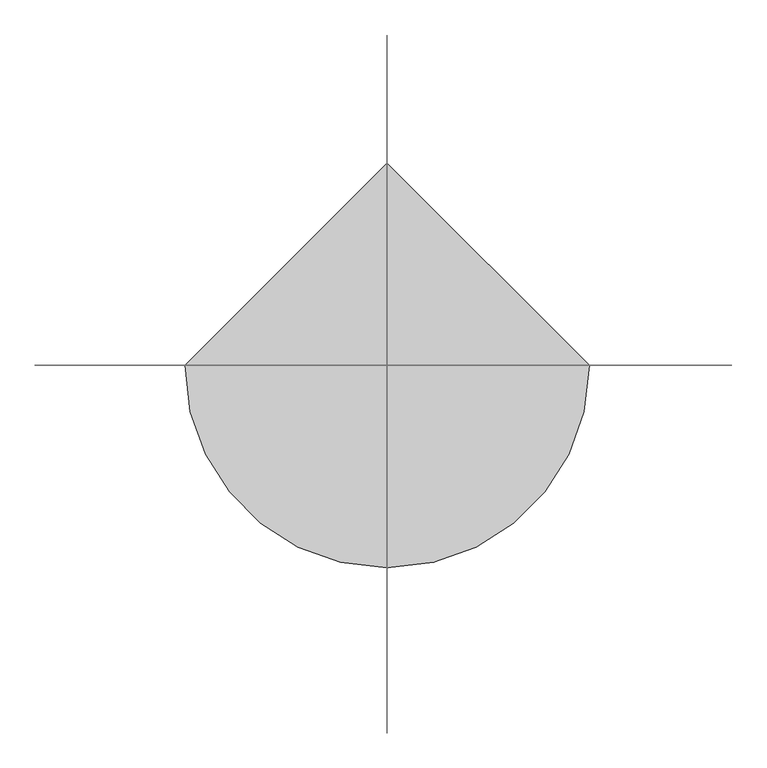
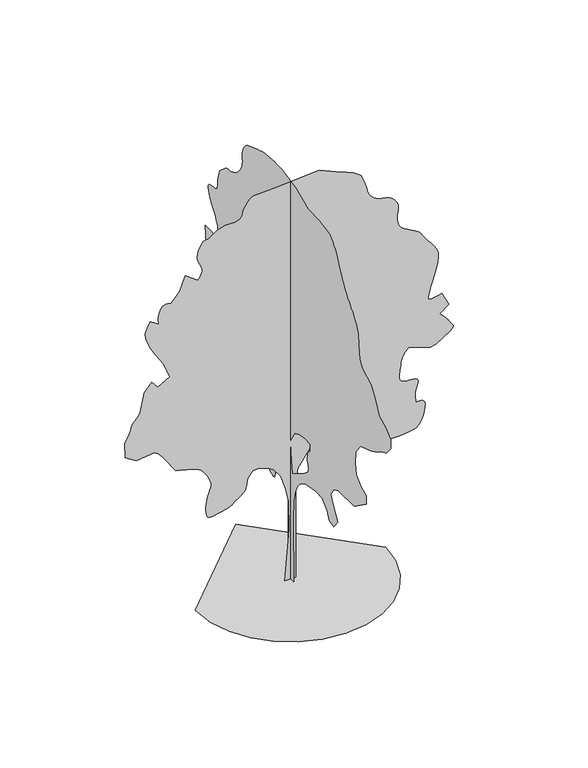
"""IFC4 building model written with IfcOpenShell, lengths in millimetres: geographic element geometry, RPC 木 - 落葉樹 : ポプラ - 7.6 メートル."""

from ifc_helpers import new_model, si_unit, origin, place, context, project, spatial, triangles, source, transform, mapped, element, save


def geographic_element_a2efc43f(model_context):
    return source(origin(), model_context, "Body", "Tessellation", [
        triangles([(92.8617737, 0.000406, 0.005513), (-103.915959, 0.000406, 0.005513), (-22.8901635, 0.0003494, 949.1680813), (-34.4652064, 0.0003176, 1481.626133), (-92.3406663, 0.0003011, 1759.4311237), (-173.3674883, 0.0002866, 2002.5093098), (-300.6936918, 0.0002762, 2176.1362118), (-404.8693279, 0.0002728, 2234.0127663), (-566.9214277, 0.0002694, 2291.8891754), (-682.6743914, 0.0002694, 2291.8891754), (-763.7004049, 0.0002762, 2176.1362118), (-798.427355, 0.0002852, 2025.6589142), (-801.2950579, 0.0002863, 2008.1460297), (-806.4934324, 0.0002874, 1989.7185207), (-816.3455927, 0.0002886, 1969.4722275), (-833.1871519, 0.0002899, 1946.489764), (-859.3387533, 0.0002915, 1919.8644997), (-897.1360102, 0.0002934, 1888.6816647), (-948.9046526, 0.0002956, 1852.0320122), (-998.3097038, 0.0002977, 1817.003627), (-1032.3247061, 0.0002993, 1790.0718407), (-1058.2431822, 0.0003005, 1769.4200489), (-1083.3510246, 0.0003015, 1753.2219097), (-1114.9365967, 0.0003023, 1739.6560226), (-1160.2933485, 0.000303, 1726.8980804), (-1226.7072453, 0.0003038, 1713.1294441), (-1299.8367931, 0.0003048, 1697.5064152), (-1361.0192505, 0.0003056, 1683.0943588), (-1411.0653236, 0.0003062, 1673.9514576), (-1450.7852829, 0.0003062, 1674.1187439), (-1480.9902706, 0.0003054, 1687.6517841), (-1502.4856155, 0.0003035, 1718.5964069), (-1516.0869656, 0.0003004, 1771.0059986), (-1522.0251205, 0.0002967, 1833.4043701), (-1521.0802654, 0.0002932, 1891.7521168), (-1514.8710514, 0.00029, 1946.2541679), (-1505.0164204, 0.0002869, 1997.1108021), (-1493.1376396, 0.0002841, 2044.5246231), (-1480.8535057, 0.0002815, 2088.6983803), (-1469.7852859, 0.000279, 2129.8370029), (-1458.1775642, 0.0002769, 2165.8103886), (-1444.9485752, 0.000275, 2196.5194153), (-1432.7328964, 0.0002733, 2225.2042923), (-1424.1600185, 0.0002715, 2255.1052288), (-1421.8648098, 0.0002695, 2289.4596725), (-1428.479377, 0.000267, 2331.5079781), (-1446.6356815, 0.0002638, 2384.4900639), (-1473.3978561, 0.0002604, 2441.7913628), (-1503.3976238, 0.0002573, 2494.2338013), (-1535.6266159, 0.0002545, 2541.2094223), (-1569.0690514, 0.0002521, 2582.1226227), (-1602.7142361, 0.00025, 2616.3228607), (-1635.5487144, 0.0002484, 2643.2520309), (-1666.5642632, 0.0002473, 2662.3026123), (-1701.7269424, 0.0002464, 2677.1732162), (-1746.6125748, 0.0002455, 2692.0694), (-1799.5946606, 0.0002446, 2706.940004), (-1859.0568741, 0.0002437, 2721.8358971), (-1923.3782387, 0.0002428, 2736.706501), (-1990.9396671, 0.000242, 2751.5771049), (-2060.1197468, 0.0002411, 2766.4732887), (-2256.8962532, 0.0002238, 3055.8556252), (-2301.7818855, 0.0002202, 3116.5289566), (-2338.160479, 0.0002175, 3161.4195305), (-2367.4508423, 0.0002156, 3193.1367805), (-2391.0741096, 0.0002144, 3214.3154297), (-2410.4440029, 0.0002136, 3227.61549), (-2426.9815109, 0.0002131, 3235.6461044), (-2442.1003555, 0.0002128, 3241.041996), (-2766.1945267, 0.0002148, 3206.3353935), (-2962.9836777, 0.0002073, 3333.6607613), (-2974.5611687, 0.0001914, 3599.8884064), (-2952.3436295, 0.000189, 3639.5351143), (-2930.8609291, 0.0001867, 3678.9789276), (-2910.7717484, 0.0001843, 3718.0428223), (-2892.8103447, 0.0001821, 3756.473616), (-2877.7118477, 0.0001798, 3794.0934128), (-2866.1343567, 0.0001776, 3830.70019), (-2858.8130013, 0.0001755, 3866.1160515), (-2847.3878265, 0.0001735, 3899.5814507), (-2825.6772331, 0.0001716, 3931.2481224), (-2797.4559906, 0.0001698, 3962.0787987), (-2766.6000252, 0.0001679, 3993.137368), (-2736.9852631, 0.000166, 4025.3865623), (-2712.4120537, 0.000164, 4059.8905609), (-2696.7560326, 0.0001617, 4097.611805), (-2627.2919586, 0.000141, 4444.881015), (-2488.4021805, 0.0001321, 4595.3354942), (-2384.2239464, 0.0001396, 4468.0101265), (-2164.2953648, 0.0001327, 4583.7832924), (-2280.0483284, 0.0001155, 4873.1403397), (-2465.2501053, 9.82e-05, 5162.5226761), (-2487.5231644, 9.58e-05, 5203.6643509), (-2513.036142, 9.27e-05, 5254.9385468), (-2539.3601166, 8.93e-05, 5312.268187), (-2564.0600624, 8.58e-05, 5371.6238663), (-2584.7067673, 8.24e-05, 5428.9535065), (-2598.8934013, 7.93e-05, 5480.2277023), (-2604.1628471, 7.69e-05, 5521.3693771), (-2601.4519661, 7.48e-05, 5555.7463486), (-2593.9027176, 7.28e-05, 5589.5407974), (-2582.2746483, 7.08e-05, 5622.8038834), (-2567.4293335, 6.89e-05, 5655.6611801), (-2550.1521904, 6.69e-05, 5688.2394241), (-2531.2585762, 6.5e-05, 5720.5903564), (-2511.5516396, 6.31e-05, 5752.8651306), (-2361.0744873, 6.93e-05, 5648.6941635), (-2365.8675087, 6.73e-05, 5681.019516), (-2369.6472198, 6.54e-05, 5713.8518143), (-2371.4003105, 6.34e-05, 5747.6968414), (-2370.118412, 6.13e-05, 5783.0621246), (-2364.7857433, 5.9e-05, 5820.4540283), (-2354.391465, 5.67e-05, 5860.3794983), (-2337.9248829, 5.41e-05, 5903.344899), (-2316.394075, 5.19e-05, 5940.9141174), (-2291.8258072, 5.04e-05, 5965.7155106), (-2264.7267345, 4.95e-05, 5979.8768555), (-2235.6036575, 4.92e-05, 5985.5515091), (-2204.9604698, 4.92e-05, 5984.8422501), (-2173.3064426, 4.95e-05, 5979.8768555), (-2141.1459057, 5e-05, 5972.7831024), (-1990.6686081, 3.96e-05, 6146.4178528), (-1886.4928448, 2.44e-05, 6401.0680069), (-1666.5642632, 3.41e-05, 6239.0110382), (-1644.4939533, 3.23e-05, 6268.8284042), (-1623.9409927, 3.05e-05, 6298.823085), (-1606.4256374, 2.87e-05, 6329.2229736), (-1593.4675621, 2.69e-05, 6360.2309647), (-1586.584552, 2.5e-05, 6392.0749512), (-1587.2913403, 2.3e-05, 6424.9066681), (-1597.1131245, 2.1e-05, 6458.9545898), (-1613.1085144, 1.89e-05, 6493.7879288), (-1630.1173599, 1.68e-05, 6529.2043716), (-1646.3153538, 1.46e-05, 6565.8614365), (-1659.8813862, 1.23e-05, 6604.3428085), (-1668.993766, 9.9e-06, 6645.2304291), (-1671.8286221, 7.3e-06, 6689.1585617), (-1666.5642632, 4.4e-06, 6736.759726), (-1653.9432312, 1.5e-06, 6785.3747818), (-1636.4607227, -1.2e-06, 6830.974324), (-1614.9299149, -3.6e-06, 6871.9131042), (-1590.1616592, -5.7e-06, 6906.5691284), (-1562.9612846, -7.3e-06, 6933.3209839), (-1534.1394974, -8.3e-06, 6950.5728378), (-1504.512236, -8.7e-06, 6956.6782791), (-1471.3382435, -9.2e-06, 6965.0132355), (-1431.8891979, -1.05e-05, 6986.521225), (-1386.9707188, -1.22e-05, 7015.9078033), (-1337.3959831, -1.41e-05, 7047.9291046), (-1283.9756973, -1.59e-05, 7077.315683), (-1227.5178062, -1.72e-05, 7098.8236725), (-1168.8306908, -1.77e-05, 7107.1580475), (-1109.0314339, -1.76e-05, 7106.8289978), (-1050.4481638, -1.77e-05, 7107.2847839), (-995.7104439, -1.79e-05, 7110.8060806), (-947.4530697, -1.84e-05, 7119.5718246), (-908.3054592, -1.94e-05, 7135.8353668), (-880.9024807, -2.09e-05, 7161.8273849), (-867.8760956, -2.32e-05, 7199.7512329), (-856.9422426, -2.61e-05, 7248.5941818), (-835.6824938, -2.93e-05, 7302.6804153), (-806.5264246, -3.26e-05, 7357.4009125), (-771.9008492, -3.56e-05, 7408.0420074), (-734.2403572, -3.81e-05, 7449.9940979), (-695.9718355, -3.98e-05, 7478.5696793), (-659.5247869, -4.04e-05, 7489.1335693), (-323.8458215, -4.18e-05, 7512.2885513), (509.5693688, -4.53e-05, 7570.1751343), (926.2744205, -3.42e-05, 7384.9631836), (995.3532709, -3.26e-05, 7357.5526474), (1062.2078384, -3.09e-05, 7329.4578506), (1124.6038118, -2.92e-05, 7299.9195374), (1180.3219225, -2.73e-05, 7268.2778641), (1227.1277138, -2.52e-05, 7233.7741562), (1262.7970482, -2.29e-05, 7195.7485703), (1285.1055702, -2.04e-05, 7153.4674301), (1299.9533558, -1.79e-05, 7111.9461273), (1314.5985374, -1.58e-05, 7075.1117477), (1328.8409821, -1.37e-05, 7040.480722), (1342.4753242, -1.16e-05, 7005.6473831), (1355.2991055, -9.4e-06, 6968.1799026), (1367.1094311, -6.8e-06, 6925.6702881), (1377.7063133, -3.9e-06, 6875.662294), (1393.5345623, -8e-07, 6823.9573105), (1419.2834267, 2e-06, 6778.1292938), (1452.117905, 4.3e-06, 6738.3811386), (1489.2059029, 6.3e-06, 6704.890741), (1527.709948, 7.9e-06, 6677.9104111), (1564.7979458, 9.1e-06, 6657.5936279), (1597.6348949, 9.9e-06, 6644.1415421), (1628.0070236, 1.04e-05, 6636.0856384), (1659.1872425, 1.07e-05, 6630.6638763), (1690.5726814, 1.1e-05, 6626.230426), (1721.5527672, 1.13e-05, 6621.2144531), (1751.5195427, 1.17e-05, 6613.9439667), (1779.8675217, 1.24e-05, 6602.8481323), (1805.9861309, 1.34e-05, 6586.2799576), (1831.2638031, 1.47e-05, 6563.7586578), (1856.5388592, 1.63e-05, 6536.6015945), (1880.3977226, 1.82e-05, 6505.7959167), (1901.4218754, 2.02e-05, 6472.3560974), (1918.1949795, 2.23e-05, 6437.2948654), (1929.2986622, 2.44e-05, 6401.625531), (1933.3139694, 2.65e-05, 6366.3364059), (1929.8053173, 2.9e-05, 6325.1191544), (1922.2457497, 3.2e-05, 6273.1351181), (1915.0916805, 3.56e-05, 6213.8805954), (1912.7964718, 3.93e-05, 6150.775145), (1919.8163921, 4.31e-05, 6087.2644867), (1940.6048035, 4.67e-05, 6026.7937592), (1979.615649, 5e-05, 5972.7831024), (2034.2165314, 5.26e-05, 5927.5631882), (2096.1082478, 5.5e-05, 5888.8289246), (2161.2401733, 5.71e-05, 5853.1340103), (2225.5615379, 5.92e-05, 5817.0088898), (2285.0238968, 6.16e-05, 5777.0584213), (2335.5764797, 6.44e-05, 5729.8118866), (2373.1711327, 6.79e-05, 5671.8491455), (2411.6421856, 7.17e-05, 5607.223439), (2462.6659607, 7.56e-05, 5541.7878983), (2518.9567108, 7.96e-05, 5474.7303635), (2573.2307236, 8.38e-05, 5405.2410004), (2618.1721664, 8.81e-05, 5332.5093933), (2646.5201454, 9.27e-05, 5255.7495438), (2650.9785942, 9.76e-05, 5174.0998764), (2634.6386032, 0.0001032, 5079.7841217), (2608.190799, 0.0001097, 4970.8762344), (2575.6628426, 0.0001165, 4855.508567), (2541.0826859, 0.0001233, 4741.7367325), (2508.5622871, 0.0001295, 4637.6927925), (2482.1043091, 0.0001347, 4551.4835197), (2465.7718758, 0.0001383, 4491.1648178), (2464.9611694, 0.0001404, 4454.9635391), (2480.5538223, 0.0001417, 4433.9369156), (2509.8113388, 0.0001422, 4425.5769608), (2550.0001648, 0.0001421, 4427.3248192), (2598.3867462, 0.0001415, 4436.6727951), (2652.2453773, 0.0001407, 4451.0876129), (2708.839888, 0.0001396, 4468.0101265), (2836.1652557, 0.0001548, 4213.3596817), (2674.1332855, 0.0001624, 4086.0346046), (2698.8841003, 0.0001637, 4063.6400414), (2723.4573097, 0.0001651, 4040.7132431), (2747.6253113, 0.0001665, 4016.7987144), (2771.1852104, 0.0001681, 3991.3386406), (2793.9344032, 0.0001697, 3963.8772354), (2815.6705765, 0.0001715, 3933.8828453), (2836.1652557, 0.0001735, 3900.8482338), (2858.1037422, 0.0001754, 3868.6749069), (2881.2584335, 0.000177, 3840.554821), (2901.1702995, 0.0001786, 3814.8921432), (2913.3811821, 0.0001801, 3790.0148827), (2913.4570496, 0.0001816, 3764.3269157), (2896.9144547, 0.0001833, 3736.232119), (2859.3199471, 0.0001852, 3704.0590828), (2604.6695023, 0.0001955, 3530.4243324), (2500.4962097, 0.0001962, 3518.8471321), (2118.5182171, 0.0001886, 3646.1722092), (2091.3836815, 0.0001903, 3618.7110947), (2065.163625, 0.000192, 3590.1349319), (2040.7651142, 0.0001938, 3559.3298355), (2019.0975414, 0.0001958, 3525.1551773), (2001.0780018, 0.0001981, 3486.5726486), (1987.6134167, 0.0002008, 3442.3913338), (1979.615649, 0.0002038, 3391.5220551), (1974.0473843, 0.0002068, 3342.1474525), (1967.6684132, 0.0002092, 3301.2848305), (1961.0868382, 0.0002113, 3266.096862), (1954.9106163, 0.0002132, 3233.7206406), (1949.7477047, 0.0002151, 3201.3699989), (1946.2035896, 0.0002172, 3166.1567413), (1944.888699, 0.0002197, 3125.2941193), (1953.8643139, 0.000222, 3086.7368797), (1977.0163891, 0.0002236, 3059.0981598), (2008.6704163, 0.0002247, 3040.5542336), (2043.1591541, 0.0002254, 3029.3316628), (2074.8131813, 0.0002257, 3023.5555618), (2097.9652565, 0.0002259, 3021.4277847), (2106.9408714, 0.0002259, 3021.1237335), (2119.5973663, 0.0002258, 3022.0103073), (2151.4868443, 0.0002258, 3022.4663841), (2193.5021576, 0.000226, 3019.2997169), (2236.5307812, 0.0002266, 3009.2421913), (2271.4578644, 0.0002278, 2989.0771431), (2289.1759689, 0.0002298, 2955.5102966), (2280.5702442, 0.0002328, 2905.3758568), (2259.8146797, 0.0002362, 2847.8691925), (2246.3499493, 0.0002394, 2794.0105614), (2238.9578133, 0.0002425, 2743.191861), (2236.4270084, 0.0002453, 2694.7799904), (2237.5416206, 0.0002481, 2648.2174255), (2241.0857357, 0.0002508, 2602.8707748), (2245.8432941, 0.0002535, 2558.1066467), (2285.1910378, 0.0002532, 2562.540097), (2322.5171024, 0.0002531, 2563.730722), (2355.7899261, 0.0002535, 2558.4106979), (2382.9903008, 0.0002544, 2543.4133575), (2402.0916058, 0.000256, 2515.4278564), (2411.0672207, 0.0002587, 2471.2540993), (2407.8954666, 0.0002625, 2407.6395229), (2395.1731327, 0.0002668, 2334.9507912), (2376.9836906, 0.0002708, 2266.9155544), (2353.5301804, 0.0002745, 2205.3632069), (2325.0124443, 0.0002777, 2152.110062), (2291.6383186, 0.0002803, 2108.9801365), (2253.6054657, 0.0002821, 2077.7999176), (2211.1189602, 0.0002832, 2060.3858643), (2171.2620907, 0.0002837, 2051.7801395), (2137.4826118, 0.000284, 2045.4011684), (2104.5113686, 0.0002843, 2040.64361), (2067.0864727, 0.0002845, 2036.8967457), (2019.9412399, 0.0002847, 2033.5578506), (1957.8137821, 0.000285, 2030.0137356), (1875.4374149, 0.0002852, 2025.6589142), (1785.9069786, 0.0002851, 2027.1105698), (1704.880965, 0.0002844, 2040.1039627), (1630.9405655, 0.000283, 2062.7139198), (1562.6724941, 0.0002812, 2093.0175934), (1498.6551807, 0.0002791, 2129.0947517), (1437.4727234, 0.0002767, 2169.0176056), (1377.7063133, 0.0002742, 2210.8631618), (1123.0508543, 0.0002597, 2453.9412025), (856.8231365, 0.0002528, 2569.6841377), (544.2937391, 0.0002542, 2546.5547356), (393.8164052, 0.0002611, 2430.7917435), (289.6407691, 0.00027, 2280.3144459), (127.5871523, 0.0002838, 2048.8109894), (92.8617737, 0.0003011, 1759.4311237), (92.8617737, 0.0003383, 1134.3723289), (-0.0023646, 90.6053344, 1.1e-05), (-0.0023646, -94.5971056, 0.0), (-0.0023646, -83.0220672, 1157.5168465), (-0.0023646, -94.5971056, 1527.9227257), (-0.0023646, -140.8980313, 1724.6992321), (-0.0023646, -210.3490428, 1875.1765297), (-0.0023646, -302.9508941, 1990.9294933), (-0.0023646, -441.8534077, 2071.9555069), (-0.0023646, -557.6038279, 2095.1051113), (-0.0023646, -789.1072117, 2141.4067909), (-0.0023646, -985.8861889, 2129.8320614), (-0.0023646, -1136.3635592, 1979.3546185), (-0.0023646, -1205.8147705, 1840.4521957), (-0.0023646, -1333.1399929, 1794.1505161), (-0.0023646, -1472.042561, 1967.7774181), (-0.0023646, -1321.5652634, 2199.2832001), (-0.0023646, -1252.1139793, 2361.3353725), (-0.0023646, -1333.1399929, 2500.2354698), (-0.0023646, -1483.6172905, 2569.6841377), (-0.0023646, -1969.7736626, 2569.6841377), (-0.0023646, -2351.7542713, 2835.9117828), (-0.0023646, -2351.7542713, 2997.9690422), (-0.0023646, -2189.7022442, 3067.4075363), (-0.0023646, -2039.2249466, 3206.3101044), (-0.0023646, -2004.5004673, 3403.0992554), (-0.0023646, -2027.6500717, 3634.5950089), (-0.0023646, -2178.1273693, 3831.3841599), (-0.0023646, -2444.3551598, 3923.9773453), (-0.0023646, -2488.9367409, 3941.4068047), (-0.0023646, -2533.110498, 3959.1147354), (-0.0023646, -2576.4735489, 3977.4307686), (-0.0023646, -2618.6279526, 3996.6839539), (-0.0023646, -2659.1612343, 4017.1280548), (-0.0023646, -2697.6678955, 4039.0918304), (-0.0023646, -2733.7427284, 4062.8799133), (-0.0023646, -2768.4493309, 4086.3386559), (-0.0023646, -2803.1812225, 4107.3652794), (-0.0023646, -2837.9131142, 4126.3652824), (-0.0023646, -2872.6450058, 4143.7438728), (-0.0023646, -2907.351899, 4159.9065491), (-0.0023646, -2942.0837906, 4175.258519), (-0.0023646, -2976.8156822, 4190.2052811), (-0.0023646, -3104.1407593, 4352.2622498), (-0.0023646, -3104.1407593, 4514.3195091), (-0.0023646, -2953.6609909, 4653.2220772), (-0.0023646, -2756.8971291, 4757.3924629), (-0.0023646, -2629.5467628, 5000.4657074), (-0.0023646, -2502.234185, 5185.6776581), (-0.0023646, -2224.4290489, 5336.1574265), (-0.0023646, -2143.4030354, 5463.4827942), (-0.0023646, -2120.2509602, 5718.1329483), (-0.0023646, -2097.1013557, 5926.4743011), (-0.0023646, -2072.264645, 5978.4327576), (-0.0023646, -2047.225185, 6029.4540619), (-0.0023646, -2021.7779011, 6078.651059), (-0.0023646, -1995.7251308, 6125.1127579), (-0.0023646, -1968.8641251, 6167.9514221), (-0.0023646, -1940.9873383, 6206.2043198), (-0.0023646, -1911.8997242, 6239.0110382), (-0.0023646, -1875.8225658, 6277.7964615), (-0.0023646, -1830.2327614, 6330.9455429), (-0.0023646, -1779.7788643, 6393.0121033), (-0.0023646, -1729.1274502, 6458.4988037), (-0.0023646, -1682.9270725, 6521.9838821), (-0.0023646, -1645.83922, 6577.9705811), (-0.0023646, -1622.5198586, 6620.9865601), (-0.0023646, -1605.6807701, 6657.1372604), (-0.0023646, -1585.6016178, 6696.1255783), (-0.0023646, -1563.2930958, 6737.9253525), (-0.0023646, -1539.7736012, 6782.5877426), (-0.0023646, -1516.0490318, 6830.0627518), (-0.0023646, -1493.1350235, 6880.3742157), (-0.0023646, -1472.042561, 6933.5238785), (-0.0023646, -1448.8245014, 6986.749118), (-0.0023646, -1419.5316673, 7037.5425293), (-0.0023646, -1385.1770782, 7086.3087387), (-0.0023646, -1346.7743351, 7133.4541168), (-0.0023646, -1305.3316612, 7179.3832901), (-0.0023646, -1261.8673084, 7224.5020477), (-0.0023646, -1217.3895727, 7269.2155975), (-0.0023646, -893.2828297, 7327.0766006), (-0.0023646, -546.029062, 7338.653801), (-0.0023646, -175.623419, 7500.711351), (-0.0023646, 264.2314734, 7593.3045364), (-0.0023646, 323.6937959, 7595.7363647), (-0.0023646, 382.7508016, 7597.8641418), (-0.0023646, 440.9996807, 7599.3843979), (-0.0023646, 498.0300296, 7599.9925003), (-0.0023646, 553.4441254, 7599.3843979), (-0.0023646, 606.831528, 7597.2566208), (-0.0023646, 657.7895004, 7593.3045364), (-0.0023646, 706.7891258, 7588.2379852), (-0.0023646, 754.9781902, 7582.5883301), (-0.0023646, 802.9670488, 7575.6974716), (-0.0023646, 851.3612606, 7566.9828873), (-0.0023646, 900.7663118, 7555.8620544), (-0.0023646, 951.7900869, 7541.6751297), (-0.0023646, 1005.0432318, 7523.8657516), (-0.0023646, 1340.7248497, 7408.1181656), (-0.0023646, 1370.3545818, 7383.1138779), (-0.0023646, 1399.173753, 7356.8683868), (-0.0023646, 1426.3741276, 7328.2166473), (-0.0023646, 1451.1425285, 7295.9418732), (-0.0023646, 1472.6733364, 7258.7778625), (-0.0023646, 1490.1558449, 7215.5595703), (-0.0023646, 1502.7768768, 7165.019632), (-0.0023646, 1507.1292274, 7116.7342072), (-0.0023646, 1503.584967, 7077.7714691), (-0.0023646, 1497.0060081, 7043.2421814), (-0.0023646, 1492.2458336, 7008.3076859), (-0.0023646, 1494.1711521, 6968.128743), (-0.0023646, 1507.6358826, 6917.7916992), (-0.0023646, 1537.5012108, 6852.5078934), (-0.0023646, 1578.4019119, 6786.1851974), (-0.0023646, 1620.9238804, 6734.4546341), (-0.0023646, 1663.8485859, 6694.8587952), (-0.0023646, 1705.9652012, 6664.9908508), (-0.0023646, 1746.0576668, 6642.4189728), (-0.0023646, 1782.9075977, 6624.7107513), (-0.0023646, 1815.3063469, 6609.4093597), (-0.0023646, 1845.0703732, 6598.3135254), (-0.0023646, 1874.8345448, 6592.8923447), (-0.0023646, 1904.598571, 6590.2826202), (-0.0023646, 1934.3652134, 6587.6984756), (-0.0023646, 1964.129385, 6582.2522964), (-0.0023646, 1993.8934113, 6571.1558807), (-0.0023646, 2023.6575829, 6551.5483566), (-0.0023646, 2197.2869556, 6401.0680069), (-0.0023646, 2266.7357689, 6181.1500351), (-0.0023646, 2264.4760231, 6146.5445892), (-0.0023646, 2263.5310226, 6112.7751389), (-0.0023646, 2265.2182743, 6080.6021027), (-0.0023646, 2270.8549942, 6050.8858932), (-0.0023646, 2281.7533115, 6024.3875107), (-0.0023646, 2299.23582, 6001.9417877), (-0.0023646, 2324.612178, 5984.3608841), (-0.0023646, 2359.9116222, 5974.3033585), (-0.0023646, 2402.9047829, 5970.5285889), (-0.0023646, 2448.5301956, 5967.9700241), (-0.0023646, 2491.7284309, 5961.5605316), (-0.0023646, 2527.4306122, 5946.2341415), (-0.0023646, 2550.5826874, 5916.92314), (-0.0023646, 2556.1053154, 5868.6127167), (-0.0023646, 2547.4413094, 5812.448703), (-0.0023646, 2532.0893394, 5762.3651321), (-0.0023646, 2511.1641632, 5717.3475311), (-0.0023646, 2485.7878052, 5676.3837524), (-0.0023646, 2457.0700813, 5638.4599045), (-0.0023646, 2426.1228424, 5602.562677), (-0.0023646, 2394.0634621, 5567.6531799), (-0.0023646, 2369.3609001, 5525.4981949), (-0.0023646, 2345.2664406, 5483.4705276), (-0.0023646, 2322.3854244, 5441.6201752), (-0.0023646, 2301.3284248, 5400.0732925), (-0.0023646, 2282.698312, 5358.9321991), (-0.0023646, 2267.1081299, 5318.2974701), (-0.0023646, 2255.160894, 5278.2708435), (-0.0023646, 2248.95168, 5240.6254669), (-0.0023646, 2249.4254883, 5206.6025436), (-0.0023646, 2255.4649452, 5175.6201324), (-0.0023646, 2265.9605255, 5147.0695496), (-0.0023646, 2279.797617, 5120.3426926), (-0.0023646, 2295.861462, 5094.8320404), (-0.0023646, 2313.0374485, 5069.9294907), (-0.0023646, 2463.5147461, 5093.0844727), (-0.0023646, 2648.7240807, 5093.0844727), (-0.0023646, 2625.5693893, 4757.3924629), (-0.0023646, 2417.2130665, 4398.5716324), (-0.0023646, 2409.7574169, 4356.4422272), (-0.0023646, 2402.1979946, 4314.642453), (-0.0023646, 2394.4358231, 4273.4252014), (-0.0023646, 2386.3697456, 4233.1451019), (-0.0023646, 2377.898315, 4194.0559181), (-0.0023646, 2368.9227001, 4156.486409), (-0.0023646, 2359.3391281, 4120.7664963), (-0.0023646, 2344.9953815, 4082.1586784), (-0.0023646, 2323.9712288, 4037.2681046), (-0.0023646, 2299.5044083, 3988.3492882), (-0.0023646, 2274.8373093, 3937.5814568), (-0.0023646, 2253.2051994, 3887.2441223), (-0.0023646, 2237.8507587, 3839.5162216), (-0.0023646, 2232.0114349, 3796.6522682), (-0.0023646, 2236.7360012, 3758.6522621), (-0.0023646, 2249.9651356, 3723.6921867), (-0.0023646, 2270.279884, 3691.2656776), (-0.0023646, 2296.2641991, 3660.865789), (-0.0023646, 2326.5020336, 3631.9602859), (-0.0023646, 2359.5747242, 3604.0936729), (-0.0023646, 2394.0634621, 3576.7337151), (-0.0023646, 2706.5853745, 3646.1722092), (-0.0023646, 2723.8372284, 3596.6458717), (-0.0023646, 2740.3798233, 3547.4991623), (-0.0023646, 2755.5039001, 3499.1884483), (-0.0023646, 2768.4746201, 3452.0686501), (-0.0023646, 2778.6333023, 3406.5699738), (-0.0023646, 2785.245108, 3363.0979179), (-0.0023646, 2787.6266487, 3322.0832703), (-0.0023646, 2774.199852, 3282.9940865), (-0.0023646, 2739.6958534, 3244.7153183), (-0.0023646, 2692.8545265, 3206.6647339), (-0.0023646, 2642.3654572, 3168.1833618), (-0.0023646, 2596.9426483, 3128.7142593), (-0.0023646, 2565.3015564, 3087.5981644), (-0.0023646, 2556.1053154, 3044.2784248), (-0.0023646, 2564.4399811, 3002.6556747), (-0.0023646, 2578.8547989, 2966.5049744), (-0.0023646, 2598.3361679, 2934.9397499), (-0.0023646, 2621.8454887, 2906.9969788), (-0.0023646, 2648.4200294, 2881.7903778), (-0.0023646, 2676.9959015, 2858.3825043), (-0.0023646, 2706.5853745, 2835.9117828), (-0.0023646, 2776.0491577, 2604.4160294), (-0.0023646, 2709.3974121, 2602.1106468), (-0.0023646, 2644.670549, 2600.945311), (-0.0023646, 2583.7946136, 2601.984201), (-0.0023646, 2528.6796638, 2606.3667824), (-0.0023646, 2481.2656975, 2615.2081032), (-0.0023646, 2443.468586, 2629.6226303), (-0.0023646, 2417.2130665, 2650.725412), (-0.0023646, 2391.9710026, 2676.8694557), (-0.0023646, 2357.0109272, 2705.4453278), (-0.0023646, 2313.9494568, 2736.0478203), (-0.0023646, 2264.407568, 2768.2973053), (-0.0023646, 2210.0068188, 2801.7371246), (-0.0023646, 2152.3684765, 2835.987941), (-0.0023646, 2093.1088669, 2870.6436745), (-0.0023646, 2090.6463718, 2833.3785072), (-0.0023646, 2088.2828533, 2795.8345779), (-0.0023646, 2086.1244095, 2757.6572571), (-0.0023646, 2084.2675461, 2718.5680733), (-0.0023646, 2082.8158905, 2678.2879738), (-0.0023646, 2081.8710354, 2636.4626198), (-0.0023646, 2081.533992, 2592.838829), (-0.0023646, 2079.9481876, 2547.390731), (-0.0023646, 2074.514217, 2502.7332825), (-0.0023646, 2064.2212406, 2462.5418404), (-0.0023646, 2048.0560936, 2430.4471424), (-0.0023646, 2025.0077911, 2410.0994019), (-0.0023646, 1994.0631683, 2405.1366234), (-0.0023646, 1954.2062988, 2419.2093109), (-0.0023646, 1909.2219807, 2445.3635284), (-0.0023646, 1863.6321762, 2473.9469582), (-0.0023646, 1817.5331005, 2504.5546829), (-0.0023646, 1771.028817, 2536.7762627), (-0.0023646, 1724.222953, 2570.216082), (-0.0023646, 1677.2144852, 2604.4921875), (-0.0023646, 1630.1020992, 2639.147921), (-0.0023646, 1352.2995792, 2720.1639061), (-0.0023646, 1074.4945158, 2627.5707207), (-0.0023646, 900.8676138, 2419.2093109), (-0.0023646, 923.2419748, 2389.5794334), (-0.0023646, 945.9203871, 2360.7602623), (-0.0023646, 969.204213, 2333.5598877), (-0.0023646, 993.4000471, 2308.7914867), (-0.0023646, 1018.8119408, 2287.2608242), (-0.0023646, 1045.7412563, 2269.7783157), (-0.0023646, 1074.4945158, 2257.1571384), (-0.0023646, 1101.897567, 2244.8731499), (-0.0023646, 1125.0471714, 2228.3379673), (-0.0023646, 1144.6551315, 2208.258815), (-0.0023646, 1161.4257648, 2185.344952), (-0.0023646, 1176.07349, 2160.305492), (-0.0023646, 1189.3025517, 2133.8473686), (-0.0023646, 1201.8222816, 2106.6798409), (-0.0023646, 1169.4919149, 2099.1888737), (-0.0023646, 1136.6573639, 2091.3937099), (-0.0023646, 1102.8070318, 2082.9907345), (-0.0023646, 1067.4417486, 2073.6756054), (-0.0023646, 1030.0497723, 2063.1471783), (-0.0023646, 990.1269911, 2051.0986404), (-0.0023646, 947.16675, 2037.2285568), (-0.0023646, 904.2091249, 2020.3237747), (-0.0023646, 864.2863438, 1999.7708141), (-0.0023646, 826.8943674, 1976.1830097), (-0.0023646, 791.5265408, 1950.1630863), (-0.0023646, 757.6786795, 1922.3217625), (-0.0023646, 724.8442011, 1893.2645245), (-0.0023646, 692.5138344, 1863.6018002), (-0.0023646, 692.5138344, 1701.5496277), (-0.0023646, 650.5998957, 1674.7216141), (-0.0023646, 610.2059223, 1650.6246838), (-0.0023646, 572.8469018, 1631.9970417), (-0.0023646, 540.0453429, 1621.5699165), (-0.0023646, 513.3187039, 1622.0765717), (-0.0023646, 494.1844431, 1636.2505611), (-0.0023646, 484.160055, 1666.8252937), (-0.0023646, 479.2682024, 1701.4811726), (-0.0023646, 474.7791232, 1728.6487003), (-0.0023646, 471.100714, 1752.1706657), (-0.0023646, 468.638328, 1775.8927643), (-0.0023646, 467.7947385, 1803.6682491), (-0.0023646, 468.9752624, 1839.3374382), (-0.0023646, 472.5852528, 1886.7512592), (-0.0023646, 475.5213744, 1938.6212036), (-0.0023646, 474.8120427, 1985.6298168), (-0.0023646, 471.0677945, 2028.5899853), (-0.0023646, 464.8915363, 2068.3100899), (-0.0023646, 456.893805, 2105.6006916), (-0.0023646, 447.6800869, 2141.2724968), (-0.0023646, 437.8608825, 2176.1311249), (-0.0023646, 241.0823958, 2187.7059998), (-0.0023646, 136.90626, 1990.9294933), (-0.0023646, 79.030296, 1655.2479481), (-0.0023646, 79.030296, 1226.9681305), (-0.0023646, 79.030296, 590.3344608), (-0.0022449, -48.2969385, 2025.6538273), (-0.0022449, -1.9959556, 2396.0597065), (-0.0022449, 9.5791312, 2615.9935204), (-0.0022449, -129.3229929, 2835.9117828), (-0.0022449, -279.801326, 2905.3758568), (-0.0022449, -453.4282099, 2928.5049683), (-0.0022449, -615.4803097, 2928.5049683), (-0.0022449, -615.4803097, 2789.62798), (-0.0022449, -534.4542598, 2720.1639061), (-0.0022449, -511.3046917, 2558.1066467), (-0.0022449, -521.1568156, 2548.0241226), (-0.0022449, -530.6061298, 2536.9279976), (-0.0022449, -539.2448104, 2523.7927528), (-0.0022449, -546.6699749, 2507.6277512), (-0.0022449, -552.4738358, 2487.4115433), (-0.0022449, -556.2535832, 2462.1366325), (-0.0022449, -557.6038279, 2430.7840405), (-0.0022449, -554.2294335, 2398.4207542), (-0.0022449, -544.7801193, 2370.3109875), (-0.0022449, -530.2691955, 2345.7427197), (-0.0022449, -511.7075014, 2324.0093079), (-0.0022449, -490.1108545, 2304.4038185), (-0.0022449, -466.4875508, 2286.2145218), (-0.0022449, -441.8534077, 2268.7320133), (-1707.3661331, 0.0, 0.0031185), (-1662.2297894, -391.2146745, 0.0030952), (-1533.678479, -750.4840605, 0.0030738), (-1332.01012, -1067.5126745, 0.0030549), (-1067.5126745, -1332.01012, 0.0030391), (-750.4840605, -1533.678479, 0.0030271), (-391.2146745, -1662.2297894, 0.0030194), (7.48e-05, -1707.3661331, 0.0030167), (391.2146745, -1662.2297894, 0.0030194), (750.4840605, -1533.678479, 0.0030271), (1067.5126745, -1332.01012, 0.0030391), (1332.01012, -1067.5126745, 0.0030549), (1533.678479, -750.4840605, 0.0030738), (1662.2297894, -391.2146745, 0.0030952), (1707.3661331, 0.0001493, 0.0031185), (-0.0002245, 1707.3661331, 0.0032203)], [[122, 123, 124], [87, 88, 89], [1, 2, 3], [329, 1, 3], [329, 3, 4], [328, 329, 4], [328, 4, 5], [105, 106, 107], [327, 328, 5], [327, 5, 6], [104, 105, 107], [238, 239, 240], [238, 240, 241], [237, 238, 241], [236, 237, 241], [103, 104, 107], [86, 87, 89], [235, 236, 241], [102, 103, 107], [101, 102, 107], [100, 101, 107], [99, 100, 107], [98, 99, 107], [97, 98, 107], [96, 97, 107], [327, 6, 7], [326, 327, 7], [95, 96, 107], [70, 71, 72], [69, 70, 72], [69, 72, 73], [69, 73, 74], [69, 74, 75], [69, 75, 76], [69, 76, 77], [69, 77, 78], [94, 95, 107], [234, 235, 241], [93, 94, 107], [69, 78, 79], [69, 79, 80], [69, 80, 81], [69, 81, 82], [69, 82, 83], [69, 83, 84], [69, 84, 85], [68, 69, 85], [325, 326, 7], [325, 7, 8], [67, 68, 85], [92, 93, 107], [91, 92, 107], [60, 61, 62], [67, 85, 86], [67, 86, 89], [67, 89, 90], [66, 67, 90], [65, 66, 90], [64, 65, 90], [63, 64, 90], [62, 63, 90], [60, 62, 90], [59, 60, 90], [58, 59, 90], [57, 58, 90], [56, 57, 90], [55, 56, 90], [54, 55, 90], [53, 54, 90], [284, 285, 286], [283, 284, 286], [282, 283, 286], [282, 286, 287], [281, 282, 287], [280, 281, 287], [279, 280, 287], [279, 287, 288], [278, 279, 288], [277, 278, 288], [277, 288, 289], [276, 277, 289], [275, 276, 289], [275, 289, 290], [52, 53, 90], [325, 8, 9], [121, 122, 124], [275, 290, 291], [30, 31, 32], [29, 30, 32], [29, 32, 33], [28, 29, 33], [28, 33, 34], [27, 28, 34], [27, 34, 35], [27, 35, 36], [26, 27, 36], [26, 36, 37], [26, 37, 38], [25, 26, 38], [25, 38, 39], [24, 25, 39], [23, 24, 39], [22, 23, 39], [21, 22, 39], [20, 21, 39], [20, 39, 40], [20, 40, 41], [20, 41, 42], [19, 20, 42], [19, 42, 43], [18, 19, 43], [18, 43, 44], [17, 18, 44], [16, 17, 44], [15, 16, 44], [14, 15, 44], [13, 14, 44], [12, 13, 44], [11, 12, 44], [11, 44, 45], [11, 45, 46], [10, 11, 46], [10, 46, 47], [10, 47, 48], [10, 48, 49], [10, 49, 50], [10, 50, 51], [252, 253, 254], [251, 252, 254], [251, 254, 255], [250, 251, 255], [249, 250, 255], [249, 255, 256], [248, 249, 256], [247, 248, 256], [246, 247, 256], [245, 246, 256], [245, 256, 257], [245, 257, 258], [244, 245, 258], [243, 244, 258], [242, 243, 258], [241, 242, 258], [234, 241, 258], [233, 234, 258], [274, 275, 291], [324, 325, 9], [51, 52, 90], [10, 51, 90], [9, 10, 90], [324, 9, 90], [323, 324, 90], [323, 90, 91], [323, 91, 107], [323, 107, 108], [323, 108, 109], [323, 109, 110], [323, 110, 111], [323, 111, 112], [323, 112, 113], [323, 113, 114], [323, 114, 115], [323, 115, 116], [323, 116, 117], [323, 117, 118], [323, 118, 119], [323, 119, 120], [323, 120, 121], [323, 121, 124], [323, 124, 125], [323, 125, 126], [323, 126, 127], [323, 127, 128], [323, 128, 129], [322, 323, 129], [322, 129, 130], [167, 168, 169], [274, 291, 292], [296, 297, 298], [296, 298, 299], [295, 296, 299], [294, 295, 299], [294, 299, 300], [293, 294, 300], [293, 300, 301], [293, 301, 302], [293, 302, 303], [293, 303, 304], [293, 304, 305], [293, 305, 306], [293, 306, 307], [293, 307, 308], [293, 308, 309], [293, 309, 310], [293, 310, 311], [293, 311, 312], [293, 312, 313], [293, 313, 314], [293, 314, 315], [293, 315, 316], [293, 316, 317], [293, 317, 318], [293, 318, 319], [292, 293, 319], [274, 292, 319], [274, 319, 320], [274, 320, 321], [274, 321, 322], [273, 274, 322], [273, 322, 130], [272, 273, 130], [271, 272, 130], [270, 271, 130], [269, 270, 130], [268, 269, 130], [267, 268, 130], [266, 267, 130], [265, 266, 130], [264, 265, 130], [263, 264, 130], [262, 263, 130], [261, 262, 130], [260, 261, 130], [259, 260, 130], [258, 259, 130], [233, 258, 130], [232, 233, 130], [231, 232, 130], [230, 231, 130], [229, 230, 130], [228, 229, 130], [227, 228, 130], [226, 227, 130], [225, 226, 130], [224, 225, 130], [223, 224, 130], [222, 223, 130], [221, 222, 130], [220, 221, 130], [219, 220, 130], [218, 219, 130], [217, 218, 130], [216, 217, 130], [215, 216, 130], [214, 215, 130], [213, 214, 130], [212, 213, 130], [211, 212, 130], [210, 211, 130], [209, 210, 130], [208, 209, 130], [207, 208, 130], [206, 207, 130], [205, 206, 130], [204, 205, 130], [203, 204, 130], [202, 203, 130], [201, 202, 130], [200, 201, 130], [199, 200, 130], [198, 199, 130], [197, 198, 130], [196, 197, 130], [195, 196, 130], [194, 195, 130], [193, 194, 130], [192, 193, 130], [191, 192, 130], [190, 191, 130], [189, 190, 130], [188, 189, 130], [187, 188, 130], [186, 187, 130], [185, 186, 130], [184, 185, 130], [183, 184, 130], [182, 183, 130], [181, 182, 130], [180, 181, 130], [179, 180, 130], [178, 179, 130], [177, 178, 130], [176, 177, 130], [175, 176, 130], [174, 175, 130], [173, 174, 130], [172, 173, 130], [171, 172, 130], [170, 171, 130], [169, 170, 130], [167, 169, 130], [167, 130, 131], [167, 131, 132], [167, 132, 133], [167, 133, 134], [167, 134, 135], [167, 135, 136], [164, 165, 166], [164, 166, 167], [163, 164, 167], [162, 163, 167], [161, 162, 167], [160, 161, 167], [159, 160, 167], [158, 159, 167], [143, 144, 145], [142, 143, 145], [141, 142, 145], [140, 141, 145], [140, 145, 146], [139, 140, 146], [138, 139, 146], [137, 138, 146], [136, 137, 146], [136, 146, 147], [136, 147, 148], [136, 148, 149], [136, 149, 150], [136, 150, 151], [136, 151, 152], [136, 152, 153], [136, 153, 154], [136, 154, 155], [136, 155, 156], [157, 158, 167], [157, 167, 136], [157, 136, 156], [634, 330, 635], [633, 634, 635], [632, 633, 635], [631, 632, 635], [540, 541, 542], [592, 593, 594], [494, 495, 496], [635, 330, 331], [635, 331, 332], [635, 332, 333], [635, 333, 334], [635, 334, 335], [658, 635, 335], [658, 335, 336], [658, 336, 337], [658, 337, 338], [540, 542, 543], [657, 658, 338], [631, 635, 636], [630, 631, 636], [518, 519, 520], [656, 657, 338], [656, 338, 339], [655, 656, 339], [654, 655, 339], [653, 654, 339], [540, 543, 544], [539, 540, 544], [518, 520, 521], [539, 544, 545], [538, 539, 545], [538, 545, 546], [538, 546, 547], [538, 547, 548], [537, 538, 548], [537, 548, 549], [536, 537, 549], [536, 549, 550], [536, 550, 551], [535, 536, 551], [535, 551, 552], [534, 535, 552], [493, 494, 496], [493, 496, 497], [343, 344, 345], [342, 343, 345], [341, 342, 345], [340, 341, 345], [340, 345, 346], [534, 552, 553], [533, 534, 553], [518, 521, 522], [350, 351, 352], [349, 350, 352], [349, 352, 353], [348, 349, 353], [533, 553, 554], [652, 653, 339], [518, 522, 523], [518, 523, 524], [533, 554, 555], [532, 533, 555], [518, 524, 525], [518, 525, 526], [518, 526, 527], [518, 527, 528], [518, 528, 529], [518, 529, 530], [518, 530, 531], [518, 531, 532], [518, 532, 555], [517, 518, 555], [516, 517, 555], [515, 516, 555], [607, 608, 609], [591, 592, 594], [591, 594, 595], [590, 591, 595], [590, 595, 596], [589, 590, 596], [588, 589, 596], [588, 596, 597], [587, 588, 597], [586, 587, 597], [586, 597, 598], [585, 586, 598], [585, 598, 599], [584, 585, 599], [584, 599, 600], [583, 584, 600], [583, 600, 601], [582, 583, 601], [514, 515, 555], [643, 644, 645], [630, 636, 637], [629, 630, 637], [581, 582, 601], [581, 601, 602], [348, 353, 354], [580, 581, 602], [580, 602, 603], [579, 580, 603], [651, 652, 339], [651, 339, 340], [651, 340, 346], [650, 651, 346], [649, 650, 346], [649, 346, 347], [648, 649, 347], [647, 648, 347], [646, 647, 347], [372, 373, 374], [371, 372, 374], [370, 371, 374], [369, 370, 374], [369, 374, 375], [368, 369, 375], [367, 368, 375], [366, 367, 375], [365, 366, 375], [364, 365, 375], [363, 364, 375], [362, 363, 375], [361, 362, 375], [360, 361, 375], [359, 360, 375], [358, 359, 375], [357, 358, 375], [356, 357, 375], [356, 375, 376], [356, 376, 377], [356, 377, 378], [645, 646, 347], [643, 645, 347], [642, 643, 347], [641, 642, 347], [641, 347, 348], [641, 348, 354], [641, 354, 355], [607, 609, 610], [513, 514, 555], [579, 603, 604], [607, 610, 611], [607, 611, 612], [607, 612, 613], [607, 613, 614], [607, 614, 615], [607, 615, 616], [607, 616, 617], [607, 617, 618], [607, 618, 619], [607, 619, 620], [607, 620, 621], [607, 621, 622], [607, 622, 623], [607, 623, 624], [606, 607, 624], [606, 624, 625], [605, 606, 625], [605, 625, 626], [604, 605, 626], [579, 604, 626], [579, 626, 627], [579, 627, 628], [579, 628, 629], [579, 629, 637], [578, 579, 637], [578, 637, 638], [355, 356, 378], [641, 355, 378], [641, 378, 379], [640, 641, 379], [639, 640, 379], [639, 379, 380], [639, 380, 381], [639, 381, 382], [639, 382, 383], [639, 383, 384], [639, 384, 385], [639, 385, 386], [639, 386, 387], [639, 387, 388], [639, 388, 389], [639, 389, 390], [639, 390, 391], [639, 391, 392], [639, 392, 393], [639, 393, 394], [639, 394, 395], [638, 639, 395], [578, 638, 395], [577, 578, 395], [577, 395, 396], [577, 396, 397], [577, 397, 398], [577, 398, 399], [577, 399, 400], [577, 400, 401], [577, 401, 402], [577, 402, 403], [577, 403, 404], [577, 404, 405], [577, 405, 406], [577, 406, 407], [577, 407, 408], [577, 408, 409], [577, 409, 410], [577, 410, 411], [577, 411, 412], [577, 412, 413], [577, 413, 414], [577, 414, 415], [577, 415, 416], [577, 416, 417], [577, 417, 418], [577, 418, 419], [577, 419, 420], [577, 420, 421], [577, 421, 422], [577, 422, 423], [577, 423, 424], [577, 424, 425], [577, 425, 426], [577, 426, 427], [577, 427, 428], [577, 428, 429], [577, 429, 430], [577, 430, 431], [577, 431, 432], [577, 432, 433], [577, 433, 434], [566, 567, 568], [566, 568, 569], [565, 566, 569], [564, 565, 569], [564, 569, 570], [563, 564, 570], [563, 570, 571], [562, 563, 571], [562, 571, 572], [561, 562, 572], [560, 561, 572], [560, 572, 573], [559, 560, 573], [559, 573, 574], [558, 559, 574], [558, 574, 575], [557, 558, 575], [556, 557, 575], [556, 575, 576], [555, 556, 576], [513, 555, 576], [513, 576, 577], [512, 513, 577], [511, 512, 577], [470, 471, 472], [469, 470, 472], [468, 469, 472], [468, 472, 473], [467, 468, 473], [467, 473, 474], [467, 474, 475], [466, 467, 475], [466, 475, 476], [466, 476, 477], [465, 466, 477], [465, 477, 478], [465, 478, 479], [464, 465, 479], [464, 479, 480], [464, 480, 481], [464, 481, 482], [463, 464, 482], [456, 457, 458], [456, 458, 459], [456, 459, 460], [510, 511, 577], [463, 482, 483], [455, 456, 460], [454, 455, 460], [453, 454, 460], [452, 453, 460], [451, 452, 460], [450, 451, 460], [450, 460, 461], [449, 450, 461], [449, 461, 462], [463, 483, 484], [492, 493, 497], [448, 449, 462], [447, 448, 462], [491, 492, 497], [462, 463, 484], [447, 462, 484], [447, 484, 485], [446, 447, 485], [446, 485, 486], [445, 446, 486], [445, 486, 487], [444, 445, 487], [444, 487, 488], [491, 497, 498], [509, 510, 577], [491, 498, 499], [491, 499, 500], [490, 491, 500], [490, 500, 501], [490, 501, 502], [490, 502, 503], [490, 503, 504], [490, 504, 505], [490, 505, 506], [490, 506, 507], [490, 507, 508], [490, 508, 509], [490, 509, 577], [489, 490, 577], [488, 489, 577], [444, 488, 577], [443, 444, 577], [442, 443, 577], [441, 442, 577], [440, 441, 577], [435, 436, 437], [434, 435, 437], [434, 437, 438], [434, 438, 439], [577, 434, 439], [440, 577, 439], [673, 674, 659], [672, 673, 659], [672, 659, 660], [671, 672, 660], [671, 660, 661], [671, 661, 662], [670, 671, 662], [669, 670, 662], [669, 662, 663], [669, 663, 664], [669, 664, 665], [669, 665, 666], [669, 666, 667], [669, 667, 668]], closed=False),
    ])


if __name__ == "__main__":
    model = new_model("IFC4")
    model_context = context("Model", 3, world=origin())
    ifc_project = project(units=[si_unit("LENGTHUNIT", "METRE", prefix="MILLI")], contexts=[model_context])
    site = spatial("IfcSite", under=ifc_project)
    building = spatial("IfcBuilding", under=site)
    placement = place(None, origin())
    geographic_element_shape = geographic_element_a2efc43f(model_context)
    element("IfcGeographicElement", 1, ObjectType="RPC 木 - 落葉樹 : ポプラ - 7.6 メートル", at=placement, inside=building, context=model_context, shape_type="MappedRepresentation", body=[
        mapped(geographic_element_shape, transform((0.0, 0.0, 0.0), x_axis=(1.0, 0.0, 0.0), y_axis=(0.0, 1.0, 0.0), z_axis=(0.0, 0.0, 1.0))),
    ])
    save(model, "model.ifc")

# Revit data of these elements
# Type "RPC 木 - 落葉樹 : ポプラ - 7.6 メートル"
#   built-in parameter 1005198 = "{2, 15},{39, RPC-16-G0VG-J3PX-MQ0P-J000-ST1L-LVER-AU},{1, 0},{1, 0},{2, 35},{1, 8},{5, Color},{1, 0},{1, 0},{3, 0.8},{3, 0.8},{3, 0.8},{1, 8},{7, BBoxMin},{1, 0},{1, 0},{1, 0},{1, 0},{1, 0},{1, 8},{7, BBoxMax},{1, 0},{1, 0},{1, 0},{1, 0},{1, 0},{2, 11},{9, RPCTypeId},{1, 0},{1, 0},{39, RPC-16-G0VG-J3PX-MQ0P-J000-ST1L-LVER-AU},{1, 6},{14, RPCPlantHeight},{1, 0},{1, 0},{7, 24.9344},{2, 11},{7, keyword},{1, 0},{1, 0},{178, :Geometry:RPC:Largetooth Aspen:Populus grandidentata:similar in form and aspect to trembling aspen; range does not extend as far west:east:or north; usually found on drier sites.},{2, 11},{8, category},{1, 0},{1, 0},{16, :Trees [General]},{2, 11},{12, LocalizedUID},{1, 0},{1, 0},{16, Largetooth Aspen},{2, 14},{6, Height},{1, 0},{1, 0},{7, 24.9344},{1, 2},{16, Cast Reflections},{1, 0},{1, 0},{1, 0},{1, 2},{12, Cast Shadows},{1, 0},{1, 0},{1, 1},{1, 2},{9, Lock View},{1, 0},{1, 0},{1, 0},{1, 4},{5, ViewC},{1, 0},{1, 0},{1, 0},{2, 11},{20, AdvancedUIDefinition},{1, 0},{1, 0},{0, },{2, 11},{10, AssetLibID},{1, 0},{1, 0},{36, 4D3F6E72-3F99-4203-98E9-AF80B3C7A7A4},{2, 11},{10, BaseSchema},{1, 0},{1, 0},{9, RPCSchema},{2, 11},{12, ExchangeGUID},{1, 0},{1, 0},{0, },{1, 2},{6, Hidden},{1, 0},{1, 0},{1, 0},{1, 4},{11, RPCCategory},{1, 0},{1, 0},{1, 0},{2, 11},{8, RPCImage},{1, 0},{1, 0},{0, },{1, 4},{13, SchemaVersion},{1, 0},{1, 0},{1, 4},{2, 11},{12, UIDefinition},{1, 0},{1, 0},{0, },{2, 11},{6, UIName},{1, 0},{1, 0},{39, RPC-16-G0VG-J3PX-MQ0P-J000-ST1L-LVER-AU},{2, 11},{11, VersionGUID},{1, 0},{1, 0},{9, RPCSchema},{2, 11},{9, assettype},{1, 0},{1, 0},{11, RPCGeometry},{2, 11},{11, description},{1, 0},{1, 0},{0, },{2, 11},{9, localname},{1, 0},{1, 0},{3, RPC},{2, 11},{9, localtype},{1, 0},{1, 0},{3, RPC},{1, 4},{8, revision},{1, 0},{1, 0},{1, 1},{2, 11},{9, thumbnail},{1, 0},{1, 0},{0, },{1, 4},{7, version},{1, 0},{1, 0},{1, 1},{1, 2},{20, RPC_Cast Reflections},{1, 0},{1, 0},{1, 1},{1, 2},{16, RPC_Cast Shadows},{1, 0},{1, 0},{1, 1},{1, 2},{13, RPC_Lock View},{1, 0},{1, 0},{1, 0},{1, 4},{9, RPC_ViewC},{1, 0},{1, 0},{1, 0},{21, assetlibrary_base.fbx},{1, 5},"
#   built-in parameter 1005195 = "RPC-16-G0VG-J3PX-MQ0P-J000-ST1L-LVER-AU"
#   Type Comments = "ポプラ"
#   Height = 7600 mm
#   Default Elevation = 0
